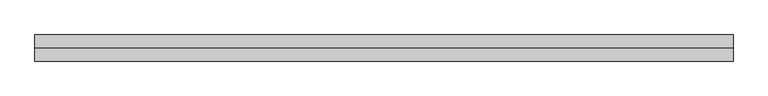
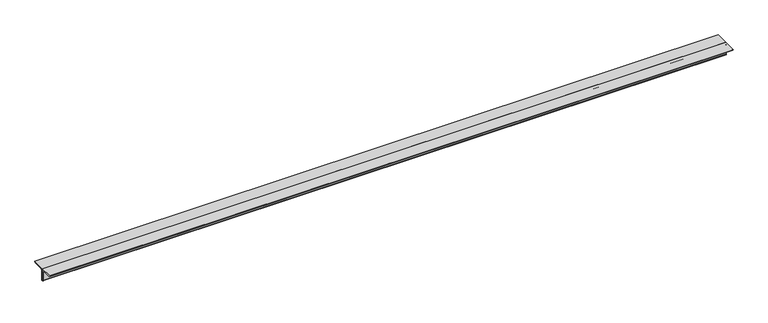
"""IFC4 building model written with IfcOpenShell, lengths in millimetres: member geometry, Steel Framing_2Ls_KS : H_SB_AR_S02_2Ls-100x100x10_VBR1."""

from ifc_helpers import new_model, si_unit, point, frame, frame_2d, origin, place, context, project, spatial, polyline, circle_curve, trimmed, segment, composite_curve, outline, extrude, source, transform, mapped, element, save


def member_50afdb99(model_context):
    return source(origin(), model_context, "Body", "SweptSolid", [
        extrude(outline(composite_curve([segment(polyline([(0.0, 28.2), (100.0, 28.2)]), True, "CONTINUOUS"), segment(trimmed(circle_curve(frame_2d((90.0, 28.2)), 10.0), [point((100.0, 28.2))], [point((90.0, 18.2))], False, "CARTESIAN"), True, "CONTINUOUS"), segment(polyline([(90.0, 18.2), (20.0, 18.2)]), True, "CONTINUOUS"), segment(trimmed(circle_curve(frame_2d((20.0, 8.2)), 10.0), [point((20.0, 18.2))], [point((10.0, 8.2))], True, "CARTESIAN"), True, "CONTINUOUS"), segment(polyline([(10.0, 8.2), (10.0, -61.8)]), True, "CONTINUOUS"), segment(trimmed(circle_curve(frame_2d((0.0, -61.8)), 10.0), [point((10.0, -61.8))], [point((0.0, -71.8))], False, "CARTESIAN"), True, "CONTINUOUS"), segment(polyline([(0.0, -71.8), (0.0, 28.2)]), True, "CONTINUOUS")], self_intersect=False)), frame((-2590.3354834, 0.0, 0.0), z_axis=(1.0, 0.0, 0.0), x_axis=(0.0, 1.0, 0.0)), (0.0, 0.0, 1.0), 5340.8352452),
        extrude(outline(composite_curve([segment(polyline([(0.0, 28.2), (0.0, -71.8)]), True, "CONTINUOUS"), segment(trimmed(circle_curve(frame_2d((0.0, -61.8)), 10.0), [point((0.0, -71.8))], [point((-10.0, -61.8))], False, "CARTESIAN"), True, "CONTINUOUS"), segment(polyline([(-10.0, -61.8), (-10.0, 8.2)]), True, "CONTINUOUS"), segment(trimmed(circle_curve(frame_2d((-20.0, 8.2)), 10.0), [point((-10.0, 8.2))], [point((-20.0, 18.2))], True, "CARTESIAN"), True, "CONTINUOUS"), segment(polyline([(-20.0, 18.2), (-90.0, 18.2)]), True, "CONTINUOUS"), segment(trimmed(circle_curve(frame_2d((-90.0, 28.2)), 10.0), [point((-90.0, 18.2))], [point((-100.0, 28.2))], False, "CARTESIAN"), True, "CONTINUOUS"), segment(polyline([(-100.0, 28.2), (0.0, 28.2)]), True, "CONTINUOUS")], self_intersect=False)), frame((-2590.3354834, 0.0, 0.0), z_axis=(1.0, 0.0, 0.0), x_axis=(0.0, 1.0, 0.0)), (0.0, 0.0, 1.0), 5340.8352452),
    ])


if __name__ == "__main__":
    model = new_model("IFC4")
    model_context = context("Model", 3, world=origin())
    ifc_project = project(units=[si_unit("LENGTHUNIT", "METRE", prefix="MILLI")], contexts=[model_context])
    site = spatial("IfcSite", under=ifc_project)
    building = spatial("IfcBuilding", under=site)
    placement = place(None, origin())
    member_shape = member_50afdb99(model_context)
    element("IfcMember", 1, ObjectType="Steel Framing_2Ls_KS : H_SB_AR_S02_2Ls-100x100x10_VBR1", at=placement, inside=building, context=model_context, shape_type="MappedRepresentation", body=[
        mapped(member_shape, transform((0.0, 0.0, 0.0), x_axis=(1.0, 0.0, 0.0), y_axis=(0.0, 1.0, 0.0), z_axis=(0.0, 0.0, 1.0))),
    ])
    save(model, "model.ifc")

# Revit data of these elements
# Type "Steel Framing_2Ls_KS : H_SB_AR_S02_2Ls-100x100x10_VBR1"
#   Type Comments = "MAIN"
#   Type Mark = "VBR1"
#   H_SectionID = "2Ls-100x100x10"
#   Assembly Code = "B10"
#   Legs = "LLBB"
#   H_Ratio for Additional Steel Plate = 0.2
#   W = 0
#   Perimeter = 0.80 m²/m
#   Nominal Weight = 29.80 kgf/m
#   Length [instance default] = 1524 mm
#   Space = 0 mm
#   b = 100 mm
#   d = 100 mm
#   t = 10 mm
#   y = 28.2 mm
#   A = 0.0038 m²
#   Structural Material [instance default] = Steel, 45-345
# Element 1 (IfcMember, "Steel Framing_2Ls_KS : H_SB_AR_S02_2Ls-100x100x10_VBR1")
#   Materials on its faces: "Steel, 45-345"
# Materials
#   "Steel, 45-345": class "Metal", colour RGB 189 187 185, transparency 0, Description = "Steel 345 MPa", Cost = 0
